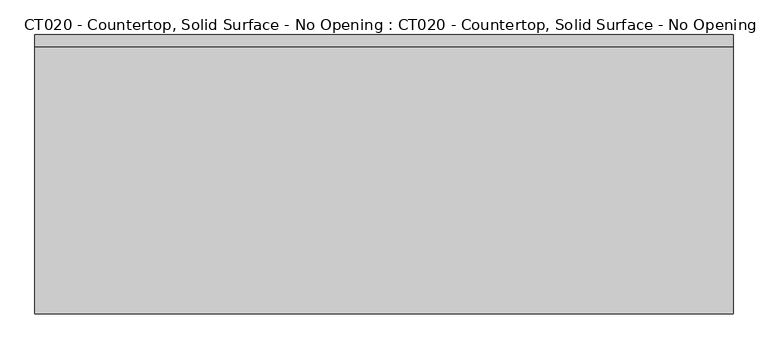
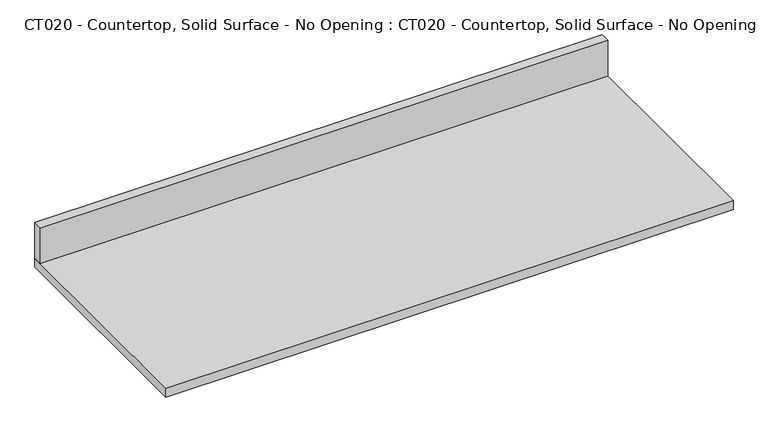
"""IFC4 building model written with IfcOpenShell, lengths in millimetres: proxy geometry, CT020 - Countertop, Solid Surface - No Opening : CT020 - Countertop, Solid Surface - No Opening."""

from ifc_helpers import new_model, si_unit, frame, origin, place, context, project, spatial, polyline, outline, extrude, source, transform, mapped, element, save


def ct020_countertop_solid_surface_no_opening_ct020_countertop_c21134b3(model_context):
    return source(origin(), model_context, "Body", "SweptSolid", [
        extrude(outline(polyline([(-762.0, 279.4), (-762.0, 304.8), (762.0, 304.8), (762.0, 279.4), (-762.0, 279.4)])), frame((0.0, 0.0, 863.6), z_axis=(0.0, 0.0, 1.0), x_axis=(1.0, 0.0, 0.0)), (0.0, 0.0, 1.0), 101.6),
        extrude(outline(polyline([(-762.0, -304.8), (-762.0, 304.8), (762.0, 304.8), (762.0, -304.8), (-762.0, -304.8)])), frame((0.0, 0.0, 838.2), z_axis=(0.0, 0.0, 1.0), x_axis=(1.0, 0.0, 0.0)), (0.0, 0.0, 1.0), 25.4),
    ])


if __name__ == "__main__":
    model = new_model("IFC4")
    model_context = context("Model", 3, world=origin())
    ifc_project = project(units=[si_unit("LENGTHUNIT", "METRE", prefix="MILLI")], contexts=[model_context])
    site = spatial("IfcSite", under=ifc_project)
    building = spatial("IfcBuilding", under=site)
    placement = place(None, origin())
    ct020_countertop_solid_surface_no_opening_ct020_countertop_shape = ct020_countertop_solid_surface_no_opening_ct020_countertop_c21134b3(model_context)
    element("IfcBuildingElementProxy", 1, Name="CT020 - Countertop, Solid Surface - No Opening : CT020 - Countertop, Solid Surface - No Opening", ObjectType="CT020 - Countertop, Solid Surface - No Opening : CT020 - Countertop, Solid Surface - No Opening", at=placement, inside=building, context=model_context, shape_type="MappedRepresentation", body=[
        mapped(ct020_countertop_solid_surface_no_opening_ct020_countertop_shape, transform((0.0, 0.0, 0.0), x_axis=(1.0, 0.0, 0.0), y_axis=(0.0, 1.0, 0.0), z_axis=(0.0, 0.0, 1.0))),
    ])
    save(model, "model.ifc")

# Revit data of these elements
# Type "CT020 - Countertop, Solid Surface - No Opening : CT020 - Countertop, Solid Surface - No Opening"
#   Watts2 = "0"
#   Watts1 = "0"
#   Unit_Issue = "LF"
#   UTIL_6_Misc = "-"
#   UTIL_5_NonMedGas = "-"
#   UTIL_4_MiscGas = "-"
#   UTIL_3_MedGas = "-"
#   UTIL_2_Elec = "-"
#   UTIL_1_WaterDrain = "-"
#   Nomenclature = "Countertop, Solid Surface"
#   NSN = ""
#   Location [instance default] = ""
#   JSN = "CT020"
#   Fund_Source_VA = "-"
#   Fund_Source_Navy = "-"
#   Fund_Source_Army = "-"
#   Fund_Source_AF = "-"
#   ELEC_Volts2 = "0"
#   ELEC_Volts1 = "0"
#   ELEC_Phase2 = "0"
#   ELEC_Phase1 = "0"
#   ELEC_HertzSwitch = "0"
#   ELEC_HertzDependent = "0"
#   ELEC_Hertz = "0"
#   ELEC_Amps2 = "0"
#   ELEC_Amps1 = "0"
#   DetailDescription = ""
#   CAT_VA = "A"
#   CAT_Navy = "A"
#   CAT_IHS = "-"
#   CAT_Army = "A"
#   CAT_AF = "A"
#   BTUperhour = "0"
#   Weight_IP = 14
#   DIM_Width_IP = 1' - 0"
#   DIM_Height_IP = 0' - 1"
#   DIM_Depth_IP = 2' - 0"
#   CustomLength [instance default] = 6' - 0"
#   Assembly Code = ""
# Element 1 (IfcBuildingElementProxy, "CT020 - Countertop, Solid Surface - No Opening : CT020 - Countertop, Solid Surface - No Opening")
#   CustomLength = 5' - 0"
#   Materials on its faces: "CounterTopFinish"
# Materials
#   "CounterTopFinish": class "Unassigned", colour RGB 139 121 96, transparency 0
